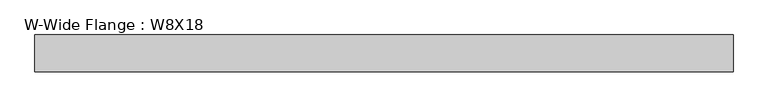
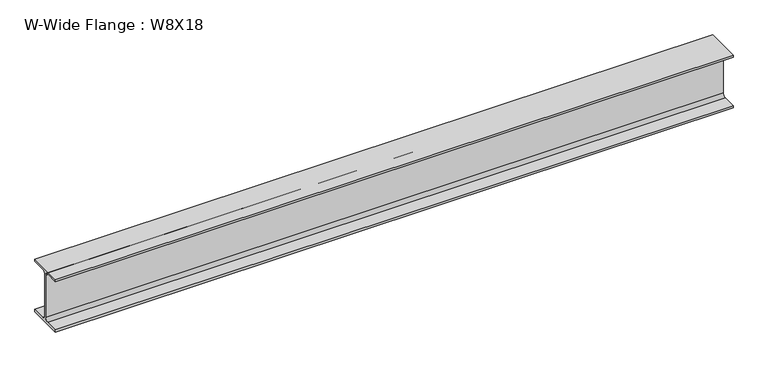
"""IFC4 building model written with IfcOpenShell, lengths in millimetres: beam geometry, W-Wide Flange : W8X18."""

from ifc_helpers import new_model, si_unit, point, frame, frame_2d, origin, place, context, project, spatial, polyline, circle_curve, trimmed, segment, composite_curve, outline, extrude, source, transform, mapped, element, save


def w_wide_flange_w8x18_db509c65(model_context):
    return source(origin(), model_context, "Body", "SweptSolid", [
        extrude(outline(composite_curve([segment(polyline([(66.675, -94.996), (66.675, -103.378), (-66.675, -103.378), (-66.675, -94.996), (-15.1765, -94.996)]), True, "CONTINUOUS"), segment(trimmed(circle_curve(frame_2d((-15.1765, -82.7405)), 12.2555), [point((-15.1765, -94.996))], [point((-2.921, -82.7405))], True, "CARTESIAN"), True, "CONTINUOUS"), segment(polyline([(-2.921, -82.7405), (-2.921, 82.7405)]), True, "CONTINUOUS"), segment(trimmed(circle_curve(frame_2d((-15.1765, 82.7405)), 12.2555), [point((-2.921, 82.7405))], [point((-15.1765, 94.996))], True, "CARTESIAN"), True, "CONTINUOUS"), segment(polyline([(-15.1765, 94.996), (-66.675, 94.996), (-66.675, 103.378), (66.675, 103.378), (66.675, 94.996), (15.1765, 94.996)]), True, "CONTINUOUS"), segment(trimmed(circle_curve(frame_2d((15.1765, 82.7405)), 12.2555), [point((15.1765, 94.996))], [point((2.921, 82.7405))], True, "CARTESIAN"), True, "CONTINUOUS"), segment(polyline([(2.921, 82.7405), (2.921, -82.7405)]), True, "CONTINUOUS"), segment(trimmed(circle_curve(frame_2d((15.1765, -82.7405)), 12.2555), [point((2.921, -82.7405))], [point((15.1765, -94.996))], True, "CARTESIAN"), True, "CONTINUOUS"), segment(polyline([(15.1765, -94.996), (66.675, -94.996)]), True, "CONTINUOUS")], self_intersect=False)), frame((-1266.825, 0.0, 0.0), z_axis=(1.0, 0.0, 0.0), x_axis=(0.0, 1.0, 0.0)), (0.0, 0.0, 1.0), 2533.65),
    ])


if __name__ == "__main__":
    model = new_model("IFC4")
    model_context = context("Model", 3, world=origin())
    ifc_project = project(units=[si_unit("LENGTHUNIT", "METRE", prefix="MILLI")], contexts=[model_context])
    site = spatial("IfcSite", under=ifc_project)
    building = spatial("IfcBuilding", under=site)
    placement = place(None, origin())
    w_wide_flange_w8x18_shape = w_wide_flange_w8x18_db509c65(model_context)
    element("IfcBeam", 1, ObjectType="W-Wide Flange : W8X18", at=placement, inside=building, context=model_context, shape_type="MappedRepresentation", body=[
        mapped(w_wide_flange_w8x18_shape, transform((0.0, 0.0, 0.0), x_axis=(1.0, 0.0, 0.0), y_axis=(0.0, 1.0, 0.0), z_axis=(0.0, 0.0, 1.0))),
    ])
    save(model, "model.ifc")

# Revit data of these elements
# Type "W-Wide Flange : W8X18"
#   Assembly Code = "B10"
#   W = 18
#   Length [instance default] = 5' - 0"
#   bf = 0' - 5 1/4"
#   d = 0' - 8.14"
#   k = 0' - 0 13/16"
#   k2 = 0' - 0.4825"
#   tf = 0' - 0.33"
#   tw = 0' - 0.23"
#   A = 0.0365278 SF
#   Structural Material [instance default] = Steel ASTM A992
# Element 1 (IfcBeam, "W-Wide Flange : W8X18")
#   Materials on its faces: "Steel ASTM A992"
# Materials
#   "Steel ASTM A992": class "Metal", colour RGB 199 199 199, transparency 0, Description = "Structural steel 50ksi", Cost = 0
